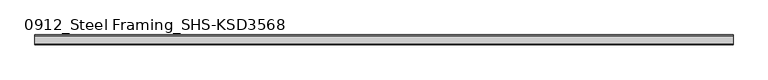
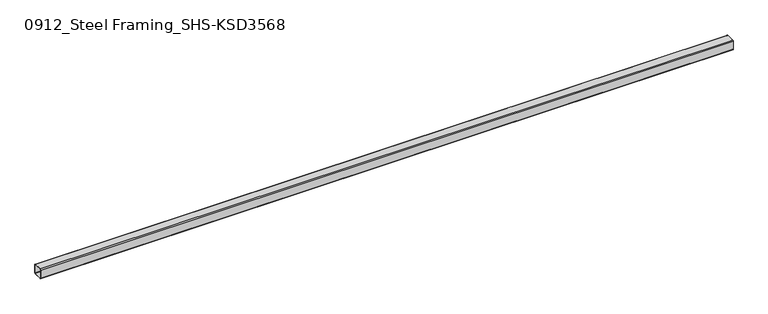
"""IFC4 building model written with IfcOpenShell, lengths in millimetres: beam geometry, 0912_Steel Framing_SHS-KSD3568 : H_SB_ASB_SHS-150x150x6."""

from ifc_helpers import new_model, si_unit, point, frame, frame_2d, origin, place, context, project, spatial, polyline, circle_curve, trimmed, segment, composite_curve, outline, extrude, source, transform, mapped, element, save


def beam_0912_steel_framing_shs_ksd3568_40d7b736(model_context):
    return source(origin(), model_context, "Body", "SweptSolid", [
        extrude(outline(composite_curve([segment(polyline([(75.0, 63.0), (75.0, -63.0)]), True, "CONTINUOUS"), segment(trimmed(circle_curve(frame_2d((63.0, -63.0)), 12.0), [point((75.0, -63.0))], [point((63.0, -75.0))], False, "CARTESIAN"), True, "CONTINUOUS"), segment(polyline([(63.0, -75.0), (-63.0, -75.0)]), True, "CONTINUOUS"), segment(trimmed(circle_curve(frame_2d((-63.0, -63.0)), 12.0), [point((-63.0, -75.0))], [point((-75.0, -63.0))], False, "CARTESIAN"), True, "CONTINUOUS"), segment(polyline([(-75.0, -63.0), (-75.0, 63.0)]), True, "CONTINUOUS"), segment(trimmed(circle_curve(frame_2d((-63.0, 63.0)), 12.0), [point((-75.0, 63.0))], [point((-63.0, 75.0))], False, "CARTESIAN"), True, "CONTINUOUS"), segment(polyline([(-63.0, 75.0), (63.0, 75.0)]), True, "CONTINUOUS"), segment(trimmed(circle_curve(frame_2d((63.0, 63.0)), 12.0), [point((63.0, 75.0))], [point((75.0, 63.0))], False, "CARTESIAN"), True, "CONTINUOUS")], self_intersect=False), holes=[composite_curve([segment(trimmed(circle_curve(frame_2d((-63.0, 63.0)), 6.0), [point((-63.0, 69.0))], [point((-69.0, 63.0))], True, "CARTESIAN"), True, "CONTINUOUS"), segment(polyline([(-69.0, 63.0), (-69.0, -63.0)]), True, "CONTINUOUS"), segment(trimmed(circle_curve(frame_2d((-63.0, -63.0)), 6.0), [point((-69.0, -63.0))], [point((-63.0, -69.0))], True, "CARTESIAN"), True, "CONTINUOUS"), segment(polyline([(-63.0, -69.0), (63.0, -69.0)]), True, "CONTINUOUS"), segment(trimmed(circle_curve(frame_2d((63.0, -63.0)), 6.0), [point((63.0, -69.0))], [point((69.0, -63.0))], True, "CARTESIAN"), True, "CONTINUOUS"), segment(polyline([(69.0, -63.0), (69.0, 63.0)]), True, "CONTINUOUS"), segment(trimmed(circle_curve(frame_2d((63.0, 63.0)), 6.0), [point((69.0, 63.0))], [point((63.0, 69.0))], True, "CARTESIAN"), True, "CONTINUOUS"), segment(polyline([(63.0, 69.0), (-63.0, 69.0)]), True, "CONTINUOUS")], self_intersect=False)]), frame((-5215.0, 0.0, 0.0), z_axis=(1.0, 0.0, 0.0), x_axis=(0.0, 1.0, 0.0)), (0.0, 0.0, 1.0), 10430.0),
    ])


if __name__ == "__main__":
    model = new_model("IFC4")
    model_context = context("Model", 3, world=origin())
    ifc_project = project(units=[si_unit("LENGTHUNIT", "METRE", prefix="MILLI")], contexts=[model_context])
    site = spatial("IfcSite", under=ifc_project)
    building = spatial("IfcBuilding", under=site)
    placement = place(None, origin())
    beam_0912_steel_framing_shs_ksd3568_shape = beam_0912_steel_framing_shs_ksd3568_40d7b736(model_context)
    element("IfcBeam", 1, ObjectType="0912_Steel Framing_SHS-KSD3568 : H_SB_ASB_SHS-150x150x6", at=placement, inside=building, context=model_context, shape_type="MappedRepresentation", body=[
        mapped(beam_0912_steel_framing_shs_ksd3568_shape, transform((0.0, 0.0, 0.0), x_axis=(1.0, 0.0, 0.0), y_axis=(0.0, 1.0, 0.0), z_axis=(0.0, 0.0, 1.0))),
    ])
    save(model, "model.ifc")

# Revit data of these elements
# Type "0912_Steel Framing_SHS-KSD3568 : H_SB_ASB_SHS-150x150x6"
#   H_WM Code_1 = "S01AA002-00001 | Main Steel Structure Fabrication Work | Shelter/Building | Medium Steel - Standard (90KG/M>Weight≥30KG/M) | Material: (   )"
#   H_WM Code_2 = "S03AA028-00001 | Main Steel Structure Erection Work | Shelter/Building | Medium Steel (90KG/M>Weight≥30KG/M) | Material: (   )"
#   H_WM Code_3 = "S01AA010-00001 | Main Steel Structure Fabrication Work | Shelter/Building | Steel Painting/Coating | for Non-Fireproofed Steel Surface, Surface Preparation, Primer, Second & Final Coat | Material: (   )"
#   H_Q'ty Cal Type Tag = "SB-Q2"
#   Perimeter = 0.60 m²/m
#   Nominal Weight = 26.40 kgf/m
#   Length [instance default] = 1.0000 m
#   b = 0.1500 m
#   h = 0.1500 m
#   tr = 0.0120 m
#   t = 0.0060 m
#   A = 28.36 m²
#   Structural Material [instance default] = Steel, 45-345
# Element 1 (IfcBeam, "0912_Steel Framing_SHS-KSD3568 : H_SB_ASB_SHS-150x150x6")
#   Structural Material = none
# Materials
#   "Steel, 45-345": class "Metal", colour RGB 189 187 185, transparency 0, Description = "Steel 345 MPa", Cost = 0
